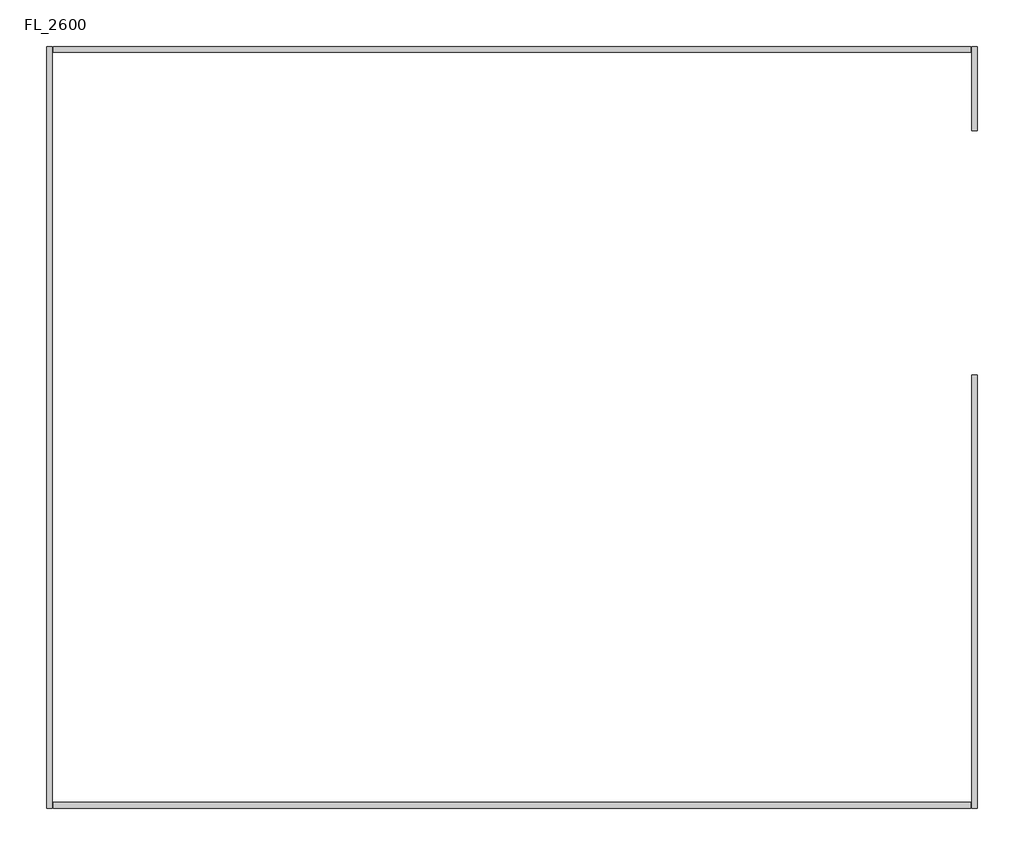
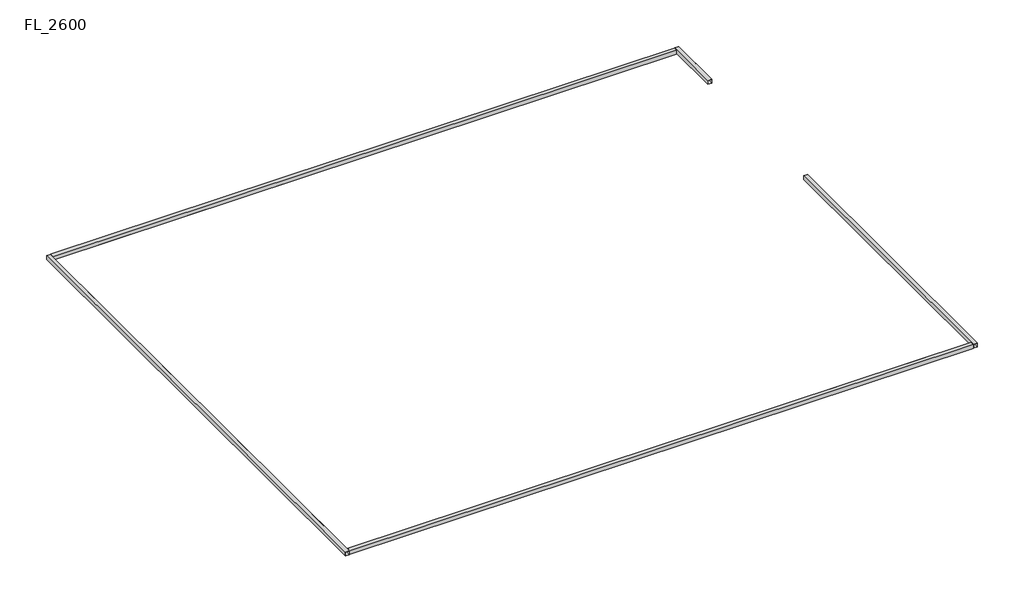
# One storey: 5 beams.
# Revit data of these elements (continued)
# Project information (continued)
#     \"af7cfdda-f71a-4a09-bb03-63e0c16d5d93-00152ffb\" ism_id=\"3a38a709-bfa8-404e-b889-5af5e78ea0bf\" /><element revit_id=\"af7cfdda-f71a-4a09-bb03-63e0c16d5d93-00152ffe\" ism_id=\"bebf0363-7e59-4a43-8f5b-502fcc4a338d\" /><element revit_id=\"af7cfdda-f71a-4a09-bb03-63e0c16d5d93-00153000\" ism_id=\"157fe154-0d28-4e8c-a143-e2896867fd28\" /><element revit_id=\"af7cfdda-f71a-4a09-bb03-63e0c16d5d93-00153002\" ism_id=\"1bf52bf8-7327-4d55-b5cd-bf7c9bf89688\" /><element revit_id=\"af7cfdda-f71a-4a09-bb03-63e0c16d5d93-00153005\" ism_id=\"7a0025bf-d54b-4614-9002-7bd4a82da90e\" /><element revit_id=\"af7cfdda-f71a-4a09-bb03-63e0c16d5d93-00153008\" ism_id=\"cad53638-8c8f-4a89-ab6f-d8a32131833b\" /><element revit_id=\"af7cfdda-f71a-4a09-bb03-63e0c16d5d93-0015300a\" ism_id=\"05672ccd-1a96-434c-8da1-7a706b3561f7\" /><element revit_id=\"af7cfdda-f71a-4a09-bb03-63e0c16d5d93-0015300c\" ism_id=\"bb809016-b2bb-4157-847e-1cca3692ba19\" /><element revit_id=\"af7cfdda-f71a-4a09-bb03-63e0c16d5d93-0015300f\" ism_id=\"720ed192-8aa7-46fd-9f7a-15d64351767c\" /><element revit_id=\"af7cfdda-f71a-4a09-bb03-63e0c16d5d93-00153011\" ism_id=\"9a47cdb9-976d-41f3-a5c3-5a7516a7763c\" /><element revit_id=\"af7cfdda-f71a-4a09-bb03-63e0c16d5d93-00153013\" ism_id=\"aba01787-c82b-453e-8db2-70277a34d5ad\" /><element revit_id=\"af7cfdda-f71a-4a09-bb03-63e0c16d5d93-00153015\" ism_id=\"f6b882e3-d64a-44b1-878c-9c00ee1fde86\" /><element revit_id=\"af7cfdda-f71a-4a09-bb03-63e0c16d5d93-00153017\" ism_id=\"95108815-490a-427a-aec1-8fcefc57c858\" /><element revit_id=\"af7cfdda-f71a-4a09-bb03-63e0c16d5d93-00153019\" ism_id=\"8fe55cf1-56b4-4a62-948a-d7f0c95bd04b\" /><element revit_id=\"af7cfdda-f71a-4a09-bb03-63e0c16d5d93-0015301b\" ism_id=\"b889bf8b-3bdd-410a-b11b-9ca69449d470\" /><element revit_id=\"af7cfdda-f71a-4a09-bb03-63e0c16d5d93-0015301d\" ism_id=\"ef8604de-de5b-45ec-9158-0b702e6ef713\" /><element revit_id=\"af7cfdda-f71a-4a09-bb03-63e0c16d5d93-0015301f\" ism_id=\"40ee286a-4bc9-4d4f-ba6d-fe1ac9da03cf\" /><element revit_id=\"af7cfdda-f71a-4a09-bb03-63e0c16d5d93-00153021\" ism_id=\"cc903f39-6bdf-4081-a56c-883169221735\" /><element revit_id=\"af7cfdda-f71a-4a09-bb03-63e0c16d5d93-00153023\" ism_id=\"0af04955-dcb6-4295-b3d4-7c432a233062\" /><element revit_id=\"af7cfdda-f71a-4a09-bb03-63e0c16d5d93-00153025\" ism_id=\"75a51549-6a04-4399-b818-f170a8c10286\" /><element revit_id=\"af7cfdda-f71a-4a09-bb03-63e0c16d5d93-00153027\" ism_id=\"7e183794-5c66-46bc-97f5-2df209b3286d\" /><element revit_id=\"af7cfdda-f71a-4a09-bb03-63e0c16d5d93-00153029\" ism_id=\"ed4a7448-29b0-44e3-8b6f-7310f83440ab\" /><element revit_id=\"af7cfdda-f71a-4a09-bb03-63e0c16d5d93-0015302b\" ism_id=\"fdb5eb17-b94e-40c1-b703-3ecb5e4efee4\" /><element revit_id=\"af7cfdda-f71a-4a09-bb03-63e0c16d5d93-0015302d\" ism_id=\"779397c1-65b7-447f-a72e-2a09308021ea\" /><element revit_id=\"af7cfdda-f71a-4a09-bb03-63e0c16d5d93-0015302f\" ism_id=\"7b409707-86c5-44e2-919e-92ad5bb9eb8b\" /><element revit_id=\"af7cfdda-f71a-4a09-bb03-63e0c16d5d93-00153031\" ism_id=\"d337c78b-590d-406c-bf20-6a3558821db1\" /><element revit_id=\"af7cfdda-f71a-4a09-bb03-63e0c16d5d93-00153033\" ism_id=\"c27f5f6d-8445-4415-853d-d316787bea6e\" /><element revit_id=\"af7cfdda-f71a-4a09-bb03-63e0c16d5d93-00153035\" ism_id=\"76036a55-3bab-417a-ba41-ec1335e2e2a7\" /><element revit_id=\"af7cfdda-f71a-4a09-bb03-63e0c16d5d93-00153037\" ism_id=\"24be638c-ff89-4616-8974-5b79c81e6e56\" /><element revit_id=\"af7cfdda-f71a-4a09-bb03-63e0c16d5d93-00153039\" ism_id=\"015f9f2c-2353-4795-b891-e4ee986f25f7\" /><element revit_id=\"af7cfdda-f71a-4a09-bb03-63e0c16d5d93-0015303b\" ism_id=\"91f8ddfb-c5b9-4f33-b141-a6edfbccf098\" /><element revit_id=\"af7cfdda-f71a-4a09-bb03-63e0c16d5d93-0015303d\" ism_id=\"78540364-1ba5-4f0c-95fb-ba8631e32695\" /><element revit_id=\"af7cfdda-f71a-4a09-bb03-63e0c16d5d93-0015303f\" ism_id=\"9d53e406-367b-4e3e-b5e8-d421731e1aab\" /><element revit_id=\"af7cfdda-f71a-4a09-bb03-63e0c16d5d93-00153041\" ism_id=\"24aa6051-1a20-4f08-8962-6f6f9ff4dc98\" /><element revit_id=\"af7cfdda-f71a-4a09-bb03-63e0c16d5d93-00153043\" ism_id=\"572a4144-5250-4962-a1b9-09502cda2774\" /><element revit_id=\"af7cfdda-f71a-4a09-bb03-63e0c16d5d93-00153045\" ism_id=\"1f486980-0be9-4aad-b32e-0608218bf68e\" /><element revit_id=\"af7cfdda-f71a-4a09-bb03-63e0c16d5d93-00153047\" ism_id=\"588ed856-d113-4521-b97c-a4d7ac7ba406\" /><element revit_id=\"af7cfdda-f71a-4a09-bb03-63e0c16d5d93-00153049\" ism_id=\"741942b7-995d-48cb-8401-4faec8ef8d15\" /><element revit_id=\"af7cfdda-f71a-4a09-bb03-63e0c16d5d93-0015304b\" ism_id=\"85254c30-08c9-46e3-acd6-6b5131f485ce\" /><element revit_id=\"af7cfdda-f71a-4a09-bb03-63e0c16d5d93-0015304e\" ism_id=\"2d57d6c0-67d8-48bd-b16f-8ef7edb485b1\" /><element revit_id=\"af7cfdda-f71a-4a09-bb03-63e0c16d5d93-00153050\" ism_id=\"57b4caff-473e-4ebc-b42c-d73ce4ca67d8\" /><element revit_id=\"af7cfdda-f71a-4a09-bb03-63e0c16d5d93-00153052\" ism_id=\"1adae240-a487-478c-a898-61bee40e7415\" /><element revit_id=\"af7cfdda-f71a-4a09-bb03-63e0c16d5d93-00153054\" ism_id=\"62613b5f-092e-4f63-86ac-d3e070a85bc5\" /><element revit_id=\"af7cfdda-f71a-4a09-bb03-63e0c16d5d93-00153056\" ism_id=\"6aecb1de-b991-4eed-80ad-e1b9ccc03a87\" /><element revit_id=\"af7cfdda-f71a-4a09-bb03-63e0c16d5d93-00153058\" ism_id=\"ecab5d8d-84d0-44a4-9549-bca959ac514b\" /><element revit_id=\"af7cfdda-f71a-4a09-bb03-63e0c16d5d93-0015305a\" ism_id=\"589f44ad-061b-46bc-91bd-bf9b1e708415\" /><element revit_id=\"af7cfdda-f71a-4a09-bb03-63e0c16d5d93-0015305c\" ism_id=\"bfa24af8-499f-45ff-9e9d-d5cc0761fed6\" /><element revit_id=\"af7cfdda-f71a-4a09-bb03-63e0c16d5d93-0015305e\" ism_id=\"8114f473-ca73-4cc8-b3e2-979f07368f66\" /><element revit_id=\"af7cfdda-f71a-4a09-bb03-63e0c16d5d93-00153060\" ism_id=\"4dde7439-2ac9-412f-a5f5-e9fd0f294ec8\" /><element revit_id=\"af7cfdda-f71a-4a09-bb03-63e0c16d5d93-00153062\" ism_id=\"661cc7d8-fd9c-4505-b43e-241bfd24b2d0\" /><element revit_id=\"af7cfdda-f71a-4a09-bb03-63e0c16d5d93-00153064\" ism_id=\"1e7f186f-1b55-4d4c-bf9f-18595049605e\" /><element revit_id=\"af7cfdda-f71a-4a09-bb03-63e0c16d5d93-00153066\" ism_id=\"ee968183-c9c6-4eab-86cf-0eda12de724b\" /><element revit_id=\"af7cfdda-f71a-4a09-bb03-63e0c16d5d93-00153068\" ism_id=\"5de1f319-cdd1-4b9a-8f8e-b86394effa22\" /><element revit_id=\"af7cfdda-f71a-4a09-bb03-63e0c16d5d93-0015306a\" ism_id=\"fa557a6c-2e39-4481-9eb5-5ede8fd31c49\" /><element revit_id=\"af7cfdda-f71a-4a09-bb03-63e0c16d5d93-0015306c\" ism_id=\"b2710e8e-0f5f-4e74-a366-aef04da22cd3\" /><element revit_id=\"af7cfdda-f71a-4a09-bb03-63e0c16d5d93-0015306e\" ism_id=\"5633c3b7-f903-46ee-b126-8a20a9a62c90\" /><element revit_id=\"af7cfdda-f71a-4a09-bb03-63e0c16d5d93-00153070\" ism_id=\"62796ef8-c4bb-4b9f-bd14-cc7392046eb4\" /><element revit_id=\"af7cfdda-f71a-4a09-bb03-63e0c16d5d93-00153072\" ism_id=\"db898ada-150e-4ff5-a9f8-16e27b46b754\" /><element revit_id=\"af7cfdda-f71a-4a09-bb03-63e0c16d5d93-00153075\" ism_id=\"d3965d2d-e119-4f6b-af8d-52c8a5397d36\" /><element revit_id=\"af7cfdda-f71a-4a09-bb03-63e0c16d5d93-00153077\" ism_id=\"063574e4-6319-4ba7-8e34-1638a1357d5f\" /><element revit_id=\"af7cfdda-f71a-4a09-bb03-63e0c16d5d93-00153079\" ism_id=\"6de69805-8980-44f0-9316-6d50d1b47cbb\" /><element revit_id=\"af7cfdda-f71a-4a09-bb03-63e0c16d5d93-0015307b\" ism_id=\"e5f77c5b-4806-4993-8875-6149db708e42\" /><element revit_id=\"af7cfdda-f71a-4a09-bb03-63e0c16d5d93-0015307d\" ism_id=\"a13071c9-c086-4896-95a6-a015bc531f25\" /><element revit_id=\"af7cfdda-f71a-4a09-bb03-63e0c16d5d93-0015307f\" ism_id=\"c9d216f9-adca-4752-b8c1-d779727505dd\" /><element revit_id=\"af7cfdda-f71a-4a09-bb03-63e0c16d5d93-00153081\" ism_id=\"5b167621-3850-4169-8bee-1e0420bf6050\" /><element revit_id=\"af7cfdda-f71a-4a09-bb03-63e0c16d5d93-00153083\" ism_id=\"09cf76ae-a083-4203-a622-7e9424374f66\" /><element revit_id=\"af7cfdda-f71a-4a09-bb03-63e0c16d5d93-00153085\" ism_id=\"14063b50-058d-464a-aa08-369865983eeb\" /><element revit_id=\"af7cfdda-f71a-4a09-bb03-63e0c16d5d93-00153087\" ism_id=\"add5837f-63be-4349-b708-9f4051059e25\" /><element revit_id=\"af7cfdda-f71a-4a09-bb03-63e0c16d5d93-00153089\" ism_id=\"b4c60bd3-61cb-423f-916a-fa2b71585228\" /><element revit_id=\"af7cfdda-f71a-4a09-bb03-63e0c16d5d93-0015308b\" ism_id=\"6251d90e-381f-4771-818c-f7465ae91864\" /><element revit_id=\"af7cfdda-f71a-4a09-bb03-63e0c16d5d93-0015308d\" ism_id=\"7693be9d-48ca-4005-bed4-90e9c08d3a38\" /><element revit_id=\"af7cfdda-f71a-4a09-bb03-63e0c16d5d93-0015308f\" ism_id=\"a6a39ca9-cd56-43ba-bfe8-2cf3b78878cc\" /><element revit_id=\"af7cfdda-f71a-4a09-bb03-63e0c16d5d93-00153091\" ism_id=\"1a3956c4-77bb-4ccc-a12d-c3514cf365d4\" /><element revit_id=\"af7cfdda-f71a-4a09-bb03-63e0c16d5d93-00153093\" ism_id=\"2ffa7a89-8ee9-470a-b3d8-7c27f566e226\" /><element revit_id=\"af7cfdda-f71a-4a09-bb03-63e0c16d5d93-00153095\" ism_id=\"e865b460-944f-4057-a6e8-4e39cb88d97d\" /><element revit_id=\"af7cfdda-f71a-4a09-bb03-63e0c16d5d93-00153097\" ism_id=\"69410bb9-8440-4a88-9151-b5459095fe2e\" /><element revit_id=\"af7cfdda-f71a-4a09-bb03-63e0c16d5d93-00153099\" ism_id=\"1efae87b-0246-432c-a428-82c87fb3929c\" /><element revit_id=\"af7cfdda-f71a-4a09-bb03-63e0c16d5d93-0015309b\" ism_id=\"e1d5fb57-3b5d-4a32-bccb-cea278671f2f\" /><element revit_id=\"af7cfdda-f71a-4a09-bb03-63e0c16d5d93-0015309d\" ism_id=\"c74a7061-f4b2-41b5-b3ff-caf6cf9dfffd\" /><element revit_id=\"af7cfdda-f71a-4a09-bb03-63e0c16d5d93-0015309f\" ism_id=\"aa777ec3-1257-49eb-b597-fbab7bda8b11\" /><element revit_id=\"af7cfdda-f71a-4a09-bb03-63e0c16d5d93-001530a1\" ism_id=\"7420a67b-bb48-477d-823a-c473ce92c083\" /><element revit_id=\"af7cfdda-f71a-4a09-bb03-63e0c16d5d93-001530a3\" ism_id=\"1ee9340a-8778-4cd6-be2d-57fb5fe16e45\" /><element revit_id=\"af7cfdda-f71a-4a09-bb03-63e0c16d5d93-001530a5\" ism_id=\"3216ac21-29b0-45a7-a070-99a114df4980\" /><element revit_id=\"af7cfdda-f71a-4a09-bb03-63e0c16d5d93-001530a7\" ism_id=\"dce9c5c3-a57a-4091-8398-cace2e63f290\" /><element revit_id=\"af7cfdda-f71a-4a09-bb03-63e0c16d5d93-001530a9\" ism_id=\"dcadcd2e-1b12-41e7-a9d5-5d99303c7e51\" /><element revit_id=\"af7cfdda-f71a-4a09-bb03-63e0c16d5d93-001530ab\" ism_id=\"ed4bf433-a5ea-40d4-8551-b735160eed03\" /><element revit_id=\"af7cfdda-f71a-4a09-bb03-63e0c16d5d93-001530ad\" ism_id=\"2cd91197-39b9-4301-8775-b1530f8812f8\" /><element revit_id=\"af7cfdda-f71a-4a09-bb03-63e0c16d5d93-001530af\" ism_id=\"53460b48-5382-4fff-98f2-ab500700bbca\" /><element revit_id=\"af7cfdda-f71a-4a09-bb03-63e0c16d5d93-001530b1\" ism_id=\"0d733cb9-b11e-45a1-89e1-53989b2ba4d5\" /><element revit_id=\"af7cfdda-f71a-4a09-bb03-63e0c16d5d93-001530b3\" ism_id=\"9b6990cb-bf48-452d-9572-952a8acd923b\" /><element revit_id=\"af7cfdda-f71a-4a09-bb03-63e0c16d5d93-001530b5\" ism_id=\"edb53df5-f0f8-45af-a38d-8c910b94c4aa\" /><element revit_id=\"af7cfdda-f71a-4a09-bb03-63e0c16d5d93-001530b7\" ism_id=\"a42a99cd-d791-460b-b7db-769eef45d4ee\" /><element revit_id=\"af7cfdda-f71a-4a09-bb03-63e0c16d5d93-001530b9\" ism_id=\"473eafff-0971-4b1a-8b61-a7662a5d0782\" /><element revit_id=\"af7cfdda-f71a-4a09-bb03-63e0c16d5d93-001530bb\" ism_id=\"b801d819-54a6-4fd3-91e7-5d49978bee50\" /><element revit_id=\"af7cfdda-f71a-4a09-bb03-63e0c16d5d93-001530bd\" ism_id=\"aa72d39c-13a9-4733-9528-98e90ae2a493\" /><element revit_id=\"af7cfdda-f71a-4a09-bb03-63e0c16d5d93-001530c0\" ism_id=\"e50950ab-c982-40e9-a130-a8fe9c5071aa\" /><element revit_id=\"af7cfdda-f71a-4a09-bb03-63e0c16d5d93-001530c3\" ism_id=\"caa8c896-9dda-4bb9-b942-fab7d7988525\" /><element revit_id=\"af7cfdda-f71a-4a09-bb03-63e0c16d5d93-001530c5\" ism_id=\"45f4fe9a-436c-4b4d-a48d-573edf59a390\" /><element revit_id=\"af7cfdda-f71a-4a09-bb03-63e0c16d5d93-001530c7\" ism_id=\"eb513efb-1058-4d3f-8f19-56219176a71a\" /><element revit_id=\"af7cfdda-f71a-4a09-bb03-63e0c16d5d93-001530c9\" ism_id=\"537abf12-3423-4f70-8613-a81d434152a6\" /><element revit_id=\"af7cfdda-f71a-4a09-bb03-63e0c16d5d93-001530cb\" ism_id=\"683f9f6d-960e-4ae9-ad7f-39eee39c3d47\" /><element revit_id=\"af7cfdda-f71a-4a09-bb03-63e0c16d5d93-001530cd\" ism_id=\"2ceed54c-aecf-4b75-a53e
#     -cfd758078946\" /><element revit_id=\"af7cfdda-f71a-4a09-bb03-63e0c16d5d93-001530cf\" ism_id=\"46a5ded9-4fed-43a0-a06e-bb0fce603002\" /><element revit_id=\"af7cfdda-f71a-4a09-bb03-63e0c16d5d93-001530d1\" ism_id=\"62d05a0c-55f2-4c29-a355-b77f91c84c50\" /><element revit_id=\"af7cfdda-f71a-4a09-bb03-63e0c16d5d93-001530d3\" ism_id=\"eac0c420-7041-45a3-ad98-0cab4f5d8155\" /><element revit_id=\"af7cfdda-f71a-4a09-bb03-63e0c16d5d93-001530d5\" ism_id=\"9f5beb51-429a-4c7b-aa2e-ad2efe601ed6\" /><element revit_id=\"af7cfdda-f71a-4a09-bb03-63e0c16d5d93-001530d7\" ism_id=\"4613af3e-a189-4781-a937-106d789655c9\" /><element revit_id=\"af7cfdda-f71a-4a09-bb03-63e0c16d5d93-001530d9\" ism_id=\"71402e21-51c1-43b7-b8cc-75d2aba247eb\" /><element revit_id=\"af7cfdda-f71a-4a09-bb03-63e0c16d5d93-001530db\" ism_id=\"89101b83-9b84-4f11-b026-90cd564a3900\" /><element revit_id=\"af7cfdda-f71a-4a09-bb03-63e0c16d5d93-001530dd\" ism_id=\"37670781-ce23-4ce1-992b-7a400613c37b\" /><element revit_id=\"af7cfdda-f71a-4a09-bb03-63e0c16d5d93-001530df\" ism_id=\"2316856d-18eb-466b-8ab8-114816378db0\" /><element revit_id=\"af7cfdda-f71a-4a09-bb03-63e0c16d5d93-001530e2\" ism_id=\"da4f1597-5b5a-43a6-aa94-e478ffd6cfc7\" /><element revit_id=\"af7cfdda-f71a-4a09-bb03-63e0c16d5d93-001530e5\" ism_id=\"60805764-efb2-4434-8d81-aed3c3ed3c1b\" /><element revit_id=\"af7cfdda-f71a-4a09-bb03-63e0c16d5d93-001530e8\" ism_id=\"34e34ebb-6481-4bfb-b3d0-cb52295ff652\" /><element revit_id=\"af7cfdda-f71a-4a09-bb03-63e0c16d5d93-001530eb\" ism_id=\"dd5c4d73-1406-4c40-a955-5f9c52d01161\" /><element revit_id=\"af7cfdda-f71a-4a09-bb03-63e0c16d5d93-001530ed\" ism_id=\"cf8abc6b-638f-4bd5-8b66-615be032e220\" /><element revit_id=\"af7cfdda-f71a-4a09-bb03-63e0c16d5d93-001530f0\" ism_id=\"56ce8857-0c24-48d5-82f2-459e263998e2\" /><element revit_id=\"af7cfdda-f71a-4a09-bb03-63e0c16d5d93-001530f2\" ism_id=\"a1f000e8-ea08-442b-8a96-da7657653fd5\" /><element revit_id=\"af7cfdda-f71a-4a09-bb03-63e0c16d5d93-001530f4\" ism_id=\"2625e954-f7fb-41eb-b9bd-1b615ef945fc\" /><element revit_id=\"af7cfdda-f71a-4a09-bb03-63e0c16d5d93-001530f6\" ism_id=\"48469362-393c-4deb-bbb2-ad00180a23fb\" /><element revit_id=\"af7cfdda-f71a-4a09-bb03-63e0c16d5d93-001530f8\" ism_id=\"8e650f6f-0906-45a9-8fb8-35680155d6db\" /><element revit_id=\"af7cfdda-f71a-4a09-bb03-63e0c16d5d93-001530fb\" ism_id=\"f84acaf6-20a1-4df6-afed-1dc07fd0b2e9\" /><element revit_id=\"af7cfdda-f71a-4a09-bb03-63e0c16d5d93-001530fe\" ism_id=\"72816c7e-9128-47f4-b46a-ee567a2a03d6\" /><element revit_id=\"af7cfdda-f71a-4a09-bb03-63e0c16d5d93-00153100\" ism_id=\"c95ab0f8-b4bf-4b7c-bd1d-0423c8ac725a\" /><element revit_id=\"af7cfdda-f71a-4a09-bb03-63e0c16d5d93-00153102\" ism_id=\"32fd4119-6673-4973-aef2-b39ef90310e5\" /><element revit_id=\"af7cfdda-f71a-4a09-bb03-63e0c16d5d93-00153104\" ism_id=\"fd2aa4a6-d123-4100-85b9-db27c20cf6bc\" /><element revit_id=\"af7cfdda-f71a-4a09-bb03-63e0c16d5d93-00153106\" ism_id=\"e00fdefa-e77c-4406-9dbe-3c9122259821\" /><element revit_id=\"af7cfdda-f71a-4a09-bb03-63e0c16d5d93-00153108\" ism_id=\"25e5b79e-07c2-4ffa-a7a9-bf039dd2ad78\" /><element revit_id=\"af7cfdda-f71a-4a09-bb03-63e0c16d5d93-0015310b\" ism_id=\"720021d4-ca74-47c0-9c64-7d0854fa39f5\" /><element revit_id=\"af7cfdda-f71a-4a09-bb03-63e0c16d5d93-0015310d\" ism_id=\"ea922120-0cff-4f8d-a5c2-2841c031873e\" /><element revit_id=\"af7cfdda-f71a-4a09-bb03-63e0c16d5d93-0015310f\" ism_id=\"9d07ca73-3a65-44fe-ab61-476d8d1352d1\" /><element revit_id=\"af7cfdda-f71a-4a09-bb03-63e0c16d5d93-00153111\" ism_id=\"68a2fb30-d213-40c7-a166-dad5a20bd269\" /><element revit_id=\"af7cfdda-f71a-4a09-bb03-63e0c16d5d93-00153113\" ism_id=\"06119775-28f9-44f0-a265-5c57029016d1\" /><element revit_id=\"af7cfdda-f71a-4a09-bb03-63e0c16d5d93-00153115\" ism_id=\"ca133383-8253-4d07-aa92-f507fbb2ee47\" /><element revit_id=\"af7cfdda-f71a-4a09-bb03-63e0c16d5d93-00153117\" ism_id=\"6f4a7c07-4bd3-4c99-b1e4-110c964ccc07\" /><element revit_id=\"af7cfdda-f71a-4a09-bb03-63e0c16d5d93-00153119\" ism_id=\"ee1f865b-98a9-4ff1-a84c-52926e8f3566\" /><element revit_id=\"af7cfdda-f71a-4a09-bb03-63e0c16d5d93-0015311b\" ism_id=\"4fd7bd5c-7c46-4e79-a72b-dab4a1d98f33\" /><element revit_id=\"af7cfdda-f71a-4a09-bb03-63e0c16d5d93-0015311e\" ism_id=\"9ca0cac6-aaff-412a-b9c1-a8be985bc44a\" /><element revit_id=\"af7cfdda-f71a-4a09-bb03-63e0c16d5d93-00153121\" ism_id=\"73123639-76b5-46f0-a49e-b26af36d93b1\" /><element revit_id=\"af7cfdda-f71a-4a09-bb03-63e0c16d5d93-00153123\" ism_id=\"f74e8cb9-a93d-4aaa-985b-c0ed9befad19\" /><element revit_id=\"af7cfdda-f71a-4a09-bb03-63e0c16d5d93-00153126\" ism_id=\"5778daa1-b4cb-4cc3-9b7d-323562a47fba\" /><element revit_id=\"af7cfdda-f71a-4a09-bb03-63e0c16d5d93-00153129\" ism_id=\"2d7457d2-8978-4c95-9056-ebbaed3263eb\" /><element revit_id=\"af7cfdda-f71a-4a09-bb03-63e0c16d5d93-0015312c\" ism_id=\"48b420ce-6767-430a-aadc-695c25361a2d\" /><element revit_id=\"af7cfdda-f71a-4a09-bb03-63e0c16d5d93-0015312e\" ism_id=\"fc34038c-136d-4d55-b951-9cc35899fd33\" /><element revit_id=\"af7cfdda-f71a-4a09-bb03-63e0c16d5d93-00153130\" ism_id=\"e7a25938-3b91-4519-a48d-86fdd79489d5\" /><element revit_id=\"af7cfdda-f71a-4a09-bb03-63e0c16d5d93-00153133\" ism_id=\"c81dfd8c-579c-4d77-ab89-bf1f415d9cc6\" /><element revit_id=\"af7cfdda-f71a-4a09-bb03-63e0c16d5d93-00153136\" ism_id=\"5756a4b4-84ca-418c-b9f6-2d2370afca2f\" /><element revit_id=\"af7cfdda-f71a-4a09-bb03-63e0c16d5d93-0015313a\" ism_id=\"09a9cede-a757-4d8e-a722-6140af98bc61\" /><element revit_id=\"af7cfdda-f71a-4a09-bb03-63e0c16d5d93-0015313d\" ism_id=\"ac9b583c-7f63-4351-8b69-3967279b234c\" /><element revit_id=\"af7cfdda-f71a-4a09-bb03-63e0c16d5d93-00153140\" ism_id=\"1a52584d-6b21-4de6-bb42-5b9bdd6f24e9\" /><element revit_id=\"af7cfdda-f71a-4a09-bb03-63e0c16d5d93-00153143\" ism_id=\"6c2e2bc0-8432-4c98-9292-cbb2182bd4b0\" /><element revit_id=\"af7cfdda-f71a-4a09-bb03-63e0c16d5d93-00153145\" ism_id=\"644bb900-7654-42c5-a9b7-996a2197f6d0\" /><element revit_id=\"af7cfdda-f71a-4a09-bb03-63e0c16d5d93-00153148\" ism_id=\"a1bca0bd-75db-464c-b27a-2a69d9b4ad3d\" /><element revit_id=\"af7cfdda-f71a-4a09-bb03-63e0c16d5d93-0015314a\" ism_id=\"ea29955b-34f2-409a-aefa-e6adfe75349e\" /><element revit_id=\"af7cfdda-f71a-4a09-bb03-63e0c16d5d93-0015314d\" ism_id=\"800fef33-e5e1-422c-b708-e9394bbeefcc\" /><element revit_id=\"af7cfdda-f71a-4a09-bb03-63e0c16d5d93-0015314f\" ism_id=\"86259dca-8773-4253-ac56-e71252267c8a\" /><element revit_id=\"af7cfdda-f71a-4a09-bb03-63e0c16d5d93-00153152\" ism_id=\"d15a0ad2-db9f-420d-bea3-41a78a0eb330\" /><element revit_id=\"af7cfdda-f71a-4a09-bb03-63e0c16d5d93-00153155\" ism_id=\"bd27f420-df49-4abe-bd96-8e48e7f4efcb\" /><element revit_id=\"af7cfdda-f71a-4a09-bb03-63e0c16d5d93-00153157\" ism_id=\"5d451f94-860d-4cc3-a4fa-51a9f3126e33\" /><element revit_id=\"af7cfdda-f71a-4a09-bb03-63e0c16d5d93-0015315a\" ism_id=\"4234158a-994a-492b-85da-6108709b7232\" /><element revit_id=\"af7cfdda-f71a-4a09-bb03-63e0c16d5d93-0015315c\" ism_id=\"ca24c92d-986b-417f-812f-024ab15e24c8\" /><element revit_id=\"af7cfdda-f71a-4a09-bb03-63e0c16d5d93-0015315f\" ism_id=\"699ec3b0-0151-4110-b054-14418651f324\" /><element revit_id=\"af7cfdda-f71a-4a09-bb03-63e0c16d5d93-00153161\" ism_id=\"38ecdeac-3d85-48dd-82c1-53fe93f49beb\" /><element revit_id=\"af7cfdda-f71a-4a09-bb03-63e0c16d5d93-00153163\" ism_id=\"1340aefd-b79c-4264-8a49-d0a0504eff8c\" /><element revit_id=\"af7cfdda-f71a-4a09-bb03-63e0c16d5d93-00153165\" ism_id=\"1b6167c2-fb26-4b8d-916b-d835d89896e7\" /><element revit_id=\"af7cfdda-f71a-4a09-bb03-63e0c16d5d93-00153167\" ism_id=\"290d3d83-57eb-4125-aecb-a977a5fcf5ca\" /><element revit_id=\"af7cfdda-f71a-4a09-bb03-63e0c16d5d93-00153169\" ism_id=\"105c9b97-1c70-4237-82ac-8404a3e8e6a6\" /><element revit_id=\"af7cfdda-f71a-4a09-bb03-63e0c16d5d93-0015316c\" ism_id=\"1726c5bb-05e2-4959-9da2-4227f0219f00\" /><element revit_id=\"af7cfdda-f71a-4a09-bb03-63e0c16d5d93-0015316e\" ism_id=\"d919ee9c-caed-4119-b451-e3644db952c8\" /><element revit_id=\"af7cfdda-f71a-4a09-bb03-63e0c16d5d93-00153170\" ism_id=\"1b1fab26-60c4-40ed-b31b-b177eda246ce\" /><element revit_id=\"af7cfdda-f71a-4a09-bb03-63e0c16d5d93-00153172\" ism_id=\"ea9b5221-a1f2-4796-8cca-f7872ab69cbd\" /><element revit_id=\"af7cfdda-f71a-4a09-bb03-63e0c16d5d93-00153174\" ism_id=\"660b40b2-06fb-4b62-b987-28a171e473fe\" /><element revit_id=\"af7cfdda-f71a-4a09-bb03-63e0c16d5d93-00153176\" ism_id=\"767be0d9-c5ba-4ad3-a52d-efd60031fc9a\" /><element revit_id=\"af7cfdda-f71a-4a09-bb03-63e0c16d5d93-00153178\" ism_id=\"6fbe93ce-4ed7-4596-88fc-71dafe48803e\" /><element revit_id=\"af7cfdda-f71a-4a09-bb03-63e0c16d5d93-0015317a\" ism_id=\"27d7b093-4eb7-47aa-b123-5388a6327d7f\" /><element revit_id=\"af7cfdda-f71a-4a09-bb03-63e0c16d5d93-0015317c\" ism_id=\"9073a947-5952-42fe-b37a-cdfed3ca30c7\" /><element revit_id=\"af7cfdda-f71a-4a09-bb03-63e0c16d5d93-0015317e\" ism_id=\"1888f060-aa3c-4494-8f30-a80ca2311216\" /><element revit_id=\"af7cfdda-f71a-4a09-bb03-63e0c16d5d93-00153181\" ism_id=\"c0491dc2-5df2-4c14-b988-e117f6f511a2\" /><element revit_id=\"af7cfdda-f71a-4a09-bb03-63e0c16d5d93-00153184\" ism_id=\"4f44b9aa-c092-46fe-bf9b-2d1be872d419\" /><element revit_id=\"af7cfdda-f71a-4a09-bb03-63e0c16d5d93-00153186\" ism_id=\"eb560801-76cf-40a8-a181-31cd32aca14f\" /><element revit_id=\"af7cfdda-f71a-4a09-bb03-63e0c16d5d93-00153189\" ism_id=\"8d1e5f00-41d5-42c1-9b4f-a8c2eb689a72\" /><element revit_id=\"af7cfdda-f71a-4a09-bb03-63e0c16d5d93-0015318b\" ism_id=\"caf6c2dc-0e9e-46a9-a3e1-71316081ff61\" /><element revit_id=\"af7cfdda-f71a-4a09-bb03-63e0c16d5d93-0015318d\" ism_id=\"4d149f88-f5b9-4943-8765-090324e0a65d\" /><element revit_id=\"af7cfdda-f71a-4a09-bb03-63e0c16d5d93-0015318f\" ism_id=\"75865cf2-3adc-4a52-a778-fc6fb65fcdcb\" /><element revit_id=\"af7cfdda-f71a-4a09-bb03-63e0c16d5d93-00153191\" ism_id=\"f9320017-2083-48f1-8aff-e6ba958fb1c5\" /><element revit_id=\"af7cfdda-f71a-4a09-bb03-63e0c16d5d93-00153193\" ism_id=\"38a61c12-98f2-47b1-843d-8351040e24d2\" /><element revit_id=\"af7cfdda-f71a-4a09-bb03-63e0c16d5d93-00153196\" ism_id=\"af709a9c-b664-480b-be0d-fb01aac630f2\" /><element revit_id=\"af7cfdda-f71a-4a09-bb03-63e0c16d5d93-00153199\" ism_id=\"a4c2867c-ca2a-4112-b86c-4e6563e3dc63\" /><element revit_id=\"14a48413-84c4-4e00-9e64-4f618415469a-0013ce74\" ism_id=\"F2ADF140-E21A-4820-8170-6F63D956DCAD\" /><element revit_id=\"14a48413-84c4-4e00-9e64-4f618415469a-0013ce74\" ism_id=\"B35A310E-4F33-462b-819C-3ADD300C0CEB\" /><element revit_id=\"14a48413-84c4-4e00-9e64-4f618415469a-0013ce74\" ism_id=\"711054EC-0DB2-46e3-AD20-004560300C00\" /><element revit_id=\"14a48413-84c4-4e00-9e64-4f618415469a-0013ce6e\" ism_id=\"B5C54EC9-8EBD-4860-AB72-EF5791AED394\" /><element revit_id=\"14a48413-84c4-4e00-9e64-4f618415469a-0013e793\" ism_id=\"0A7B8D02-9EA4-4aa9-A41A-E30BB5B6B6C5\" /><element revit_id=\"14a48413-84c4-4e00-9e64-4f618415469a-0013e793\" ism_id=\"714BBD27-DB58-47da-B54C-5806291C2D3C\" /><element revit_id=\"14a48413-84c4-4e00-9e64-4f618415469a-0013e793\" ism_id=\"F36E62C1-13EE-4807-A3C1-899E23E0BEDE\" /><element revit_id=\"14a48413-84c4-4e00-9e64-4f618415469a-0013e793\" ism_id=\"F5448801-679E-44d6-8F46-E676344F8165\" /><element revit_id=\"14a48413-84c4-4e00-9e64-4f618415469a-0013e793\" ism_id=\"846DCB0C-E06B-4978-9D43-E1CC0FDE7595\" /><element revit_id=\"14a48413-84c4-4e00-9e64-4f618415469a-0013e793\" ism_id=\"2ADF82B8-986D-4f44-85DE-89D921292160\" /><element revit_id=\"14a48413-84c4-4e00-9e64-4f618415469a-0013e793\" ism_id=\"7AF371ED-051B-4a30-8826-11F11C212B73\" /><element revit_id=\"14a48413-84c4-4e00-9e64-4f618415469a-0013e793\" ism_id=\"2FE74006-ADDA-412f-A522-853919E62B4D\" /><element revit_id=\"14a48413-84c4-4e00-9e64-4f618415469a-0013e793\" ism_id=\"09B63641-D581-4a6c-A18E-54C17EC989A4\" /><element revit_id=\"14a48413-84c4-4e00-9e64-4f618415469a-0013e793\" ism_id=\"0DD6B52A-77D0-45a1-82B1-8236ED57078C\" /><element revit_id=\"14a48413-84c4-4e00-9e64-4f618415469a-0013e793\" ism_id=\"35D311D2-DEB8-4469-97DE-110B6DF5B84D\" /><element revit_id=\"14a48413-84c4-4e00-9e64-4f618415469a-0013e79
#     3\" ism_id=\"0D3CCDE5-CFF9-431b-A4BD-01BF6636D6BD\" /><element revit_id=\"14a48413-84c4-4e00-9e64-4f618415469a-0013e793\" ism_id=\"C62B2A5B-024A-47ac-B030-C17A67E64A7B\" /><element revit_id=\"14a48413-84c4-4e00-9e64-4f618415469a-0013e793\" ism_id=\"944C6E43-E607-48c3-8358-9E6CB88346E7\" /><element revit_id=\"14a48413-84c4-4e00-9e64-4f618415469a-0013e793\" ism_id=\"A4B1F42D-B1C2-4ad2-8AD6-DB0D5E05998D\" /><element revit_id=\"14a48413-84c4-4e00-9e64-4f618415469a-0013e793\" ism_id=\"007E6C70-1139-4b48-B003-C76FAD4C249A\" /><element revit_id=\"14a48413-84c4-4e00-9e64-4f618415469a-0013e793\" ism_id=\"9941AC94-F03A-464c-9912-04590E0C31E0\" /><element revit_id=\"14a48413-84c4-4e00-9e64-4f618415469a-0013e793\" ism_id=\"CFD98B8D-8FF4-4e71-A909-0FE7DBCE924E\" /><element revit_id=\"14a48413-84c4-4e00-9e64-4f618415469a-0013e793\" ism_id=\"58262161-98E6-45c8-B2BD-4508105FF662\" /><element revit_id=\"14a48413-84c4-4e00-9e64-4f618415469a-0013e793\" ism_id=\"66AB4841-610A-4883-97F7-1282A56484E1\" /><element revit_id=\"14a48413-84c4-4e00-9e64-4f618415469a-0013e793\" ism_id=\"D2B324BE-BBD6-49da-9730-60EA7AD4D3A0\" /><element revit_id=\"14a48413-84c4-4e00-9e64-4f618415469a-0013e793\" ism_id=\"92A8ECE7-C053-46b1-92ED-F2C041617E7B\" /><element revit_id=\"14a48413-84c4-4e00-9e64-4f618415469a-0013e793\" ism_id=\"B4C4BDB0-65C4-4016-9C78-DBD77E229523\" /><element revit_id=\"14a48413-84c4-4e00-9e64-4f618415469a-0013e793\" ism_id=\"57270646-162F-4c83-BDB7-A5FBEA9120BD\" /><element revit_id=\"14a48413-84c4-4e00-9e64-4f618415469a-0013e793\" ism_id=\"BDEF733F-00AA-4eee-B6C6-50229FC1D236\" /><element revit_id=\"14a48413-84c4-4e00-9e64-4f618415469a-0013e793\" ism_id=\"84A94E1E-3074-40f4-9690-97191755F019\" /><element revit_id=\"14a48413-84c4-4e00-9e64-4f618415469a-0013e793\" ism_id=\"8A7D913D-7967-4718-912D-B83DF0AD2EDD\" /><element revit_id=\"14a48413-84c4-4e00-9e64-4f618415469a-0013e793\" ism_id=\"83553D70-90FA-469c-B5C3-EF03F3FC6475\" /><element revit_id=\"14a48413-84c4-4e00-9e64-4f618415469a-0013e793\" ism_id=\"6880C1E4-C50B-4c1b-B61C-23F2D8C46873\" /><element revit_id=\"14a48413-84c4-4e00-9e64-4f618415469a-0013e793\" ism_id=\"08594C43-CD40-47de-A3BA-8BFB47F64994\" /><element revit_id=\"14a48413-84c4-4e00-9e64-4f618415469a-0013e793\" ism_id=\"7D2E11FA-A5E1-4434-B9BE-AABA1A16CA03\" /><element revit_id=\"14a48413-84c4-4e00-9e64-4f618415469a-0013e793\" ism_id=\"D892DFA4-5441-4ad2-A390-253492293B1B\" /><element revit_id=\"14a48413-84c4-4e00-9e64-4f618415469a-0013e793\" ism_id=\"E5A32FE6-89C4-49f1-B3B9-1CABE7C48A4D\" /><element revit_id=\"14a48413-84c4-4e00-9e64-4f618415469a-0013e793\" ism_id=\"8AE872C2-5DBE-47c5-934B-7E964A84B589\" /><element revit_id=\"14a48413-84c4-4e00-9e64-4f618415469a-0013e793\" ism_id=\"3C847B60-488A-4604-A400-16A3A65E919B\" /><element revit_id=\"14a48413-84c4-4e00-9e64-4f618415469a-0013e793\" ism_id=\"DBEC432A-3F7B-4266-AD99-2A937DC70BCF\" /><element revit_id=\"14a48413-84c4-4e00-9e64-4f618415469a-0013e793\" ism_id=\"59403DD6-7A51-48aa-A3BE-962457E6F10E\" /><element revit_id=\"14a48413-84c4-4e00-9e64-4f618415469a-0013e793\" ism_id=\"11CDDF5D-38B6-43b2-A291-FC188BE232BC\" /><element revit_id=\"14a48413-84c4-4e00-9e64-4f618415469a-0013e793\" ism_id=\"10BF2843-EFC9-4136-933C-5B270D970277\" /><element revit_id=\"14a48413-84c4-4e00-9e64-4f618415469a-0013e793\" ism_id=\"E1B09A9C-F6C6-47d9-976B-E313C0E3F52B\" /><element revit_id=\"14a48413-84c4-4e00-9e64-4f618415469a-0013e793\" ism_id=\"A3A22EC3-26C8-4588-A0AB-AFAE02DF267E\" /><element revit_id=\"14a48413-84c4-4e00-9e64-4f618415469a-0013e793\" ism_id=\"114828FC-BDC1-4343-9119-BCB5395DAA64\" /><element revit_id=\"14a48413-84c4-4e00-9e64-4f618415469a-0013e793\" ism_id=\"797626F9-3558-4623-826F-15FB93088CB3\" /><element revit_id=\"14a48413-84c4-4e00-9e64-4f618415469a-0013e793\" ism_id=\"4BF369CD-DF09-4346-96CB-C6C6380A2599\" /><element revit_id=\"14a48413-84c4-4e00-9e64-4f618415469a-0013e793\" ism_id=\"722B46BA-61C4-44a1-9ECF-325B60B6688D\" /><element revit_id=\"14a48413-84c4-4e00-9e64-4f618415469a-0013e793\" ism_id=\"C33DBE84-19C1-4379-AB6E-A41F7420F18C\" /><element revit_id=\"14a48413-84c4-4e00-9e64-4f618415469a-0013e793\" ism_id=\"1F2D3B75-66F2-4d88-A1DD-647969477B86\" /><element revit_id=\"14a48413-84c4-4e00-9e64-4f618415469a-0013e793\" ism_id=\"DFBF96B2-410A-4f39-80C4-D8CF78561C93\" /><element revit_id=\"14a48413-84c4-4e00-9e64-4f618415469a-0013e793\" ism_id=\"D6793CD3-AB64-417c-9C28-8B18A0A2D336\" /><element revit_id=\"14a48413-84c4-4e00-9e64-4f618415469a-0013e793\" ism_id=\"90884AC0-EA00-4caa-86E1-E6B886FD90ED\" /><element revit_id=\"14a48413-84c4-4e00-9e64-4f618415469a-0013e793\" ism_id=\"64BC7B89-F7C8-4dae-A5C8-F10DF9E5F6BA\" /><element revit_id=\"14a48413-84c4-4e00-9e64-4f618415469a-0013e793\" ism_id=\"D82E4D85-2728-40e5-9F60-1C7FB2990D78\" /><element revit_id=\"14a48413-84c4-4e00-9e64-4f618415469a-0013e793\" ism_id=\"1E6D05B9-BF84-4669-AA27-948ADA1D511E\" /><element revit_id=\"14a48413-84c4-4e00-9e64-4f618415469a-0013e793\" ism_id=\"73608CB2-EB94-466e-883D-814030EF49D6\" /><element revit_id=\"14a48413-84c4-4e00-9e64-4f618415469a-0013e793\" ism_id=\"4EAF07EF-4E08-4065-9F08-BF69D4413867\" /><element revit_id=\"14a48413-84c4-4e00-9e64-4f618415469a-0013e0e9\" ism_id=\"05D74241-6318-4cac-95F5-7B878260D5B5\" /></element_binding><reinforcement_properties /><operation_settings><coordinate_mapping x=\"0\" y=\"0\" z=\"0\" /></operation_settings></ism>"
#   Building Name = "FIRE WATER PUMP BUILDING"
#   Project Status = "Project Status"
#   Client Name = "현대엔지니어링"
#   Project Address = "서울시 종로구 율곡로 75(계동)"
#   Project Name = "TAKHIATASH POWER PLANT EFFICIENCY IMPROVEMENT PROJECT / 우즈베키스탄"
#   Project Number = "BEUZ1602"
#   F01) Building Name = "FIRE WATER PUMP BUILDING"
#   F11) Project Building Tag_Type-1 = "BI aWBS"
#   F12) Project Building Tag_Type-2 = "BI aWBS"
#   F13) Project Facility Code = "621"
#   F21) Structural Type = "STEEL"
#   F31) Standard Building Code = "E204"
#   F41) Discipline = "Architecture"
#   F51) Plan Start Date-Engineering = "2018-01-01"
#   F52) Plan Finish Date-Engineering = "2018-09-13"
#   F53) Duration = "255"
#   F61) Plan Start Date-Construction = "2018-09-14"
#   F62) Plan Finish Date-Construction = "2019-12-02"
#   F63) Duration = "444"
#   F91) Plant Type = "2GTG+2STG+1HRSG"
#   F92) KKS Structures, Building = "UAB"
#   P01) Project Name = "TAKHIATASH POWER PLANT EFFICIENCY IMPROVEMENT PROJECT / 우즈베키스탄"
#   P02) Project Configuration = "2 GTG + 2 HRSG + 2STG, 2 x 250MW"
#   P03) Project Abbreviation = "UTCC"
#   P04) Project Code = "BEUZ1602"
#   P05) Project Stage = "실행"
#   P06) Project Location = "Takhiatash / Uzbekistan"
#   P07) Project Owner = "우즈베키스탄 전력청"
#   P08) Project O.E = "GAS Natural Fenosa"
#   P09) Project Schedule = "2017.10.01 ~ 2020.08.08"
#   P10) Basic Wind Speed = "48m/sec_ASCE7-05"
#   P11) Seismic = "SDS_0.15_ASCE7-05"
#   P12) Soil = "SD_ASCE7-05"
#   P13) Soil Capacity = "400 kN/m2_Soil Replacement"
#   P14) Pile Capacity = "1000 kN_D600 Board Pile"
# Grids (mm)
#   "B": line (-4148.791, 16594.538) -> (16088.062, 16594.538)
#   "A": line (-4148.791, 10594.538) -> (16088.062, 10594.538)
#   "2": line (5600, 25626.165) -> (5600, 7564.813)
#   "1": line (13600, 25626.165) -> (13600, 7564.813)
#   "3": line (-1400, 25626.165) -> (-1400, 7564.813)
#   "5": line (16088.062, 19594.538) -> (-4148.791, 19594.538)
#   "6": line (16088.062, 13594.538) -> (-4148.791, 13594.538)
#   "10": line (2100, 25626.165) -> (2100, 7564.813)
#   "12": line (9600, 25626.165) -> (9600, 7564.813)
#   "13": line (-1900, 25626.165) -> (-1900, 7564.813)
#   "14": line (14100, 25626.165) -> (14100, 7564.813)
#   "15": line (-4148.791, 23144.538) -> (16088.062, 23144.538)
#   "16": line (-4148.791, 10044.538) -> (16088.062, 10044.538)
#   "C": line (-4148.791, 22594.538) -> (16088.062, 22594.538)
# Type "Steel-Rectangular-Beam : BM125_RT-100x100x4.0"
#   t = 4 mm
#   Mass per Unit Length = 11.70 kg/m
#   Surface Area = 0.386 m²/m
#   Sectional Area = 14.95 cm²
#   Length [instance default] = 3000 mm
#   H = 100 mm
#   B = 100 mm
#   hec_material4 [instance default] = none
#   hec_material3 [instance default] = none
#   hec_material2 [instance default] = none
#   hec_material1 [instance default] = none
#   Structural Material [instance default] = none
# Elements 1, 2, 3, 4, 5 (IfcBeam, "Steel-Rectangular-Beam : BM125_RT-100x100x4.0")
#   Comments = ""
#   F01) Building Name = "Fire Water Pump Building"
#   F11) Project Building Tag_Type-1 = ""
#   F12) Project Building Tag_Type-2 = ""
#   F13) Project Facility Code = "621"
#   F21) Structural Type = "Steel"
#   F31) Standard Building Code = "E204"
#   F41) Discipline = "Architecture"
#   F51) Plan Start Date-Engineering = "2018-09-14"
#   F52) Plan Finish Date-Engineering = "2019-12-02"
#   F53) Duration = "444"
#   W11) Activity ID = "T3C621AR4110"
#   W12) Activity Name = "Fire Water Pump BLDG - Main Steel Structure"
#   W13) Plan Start Date = "2019-04-02"
#   W14) Plan Finish Date = "2019-06-03"
#   hec_material4 = none
#   hec_material3 = none
#   hec_material2 = S01AA010-00001_Main Steel Structure Fabrication Work_Shelter/Building_Steel Painting/Coating_for Non-Fireproofed Steel Surface, Surface Preparation, Primer, Second & Final Coat
#   hec_material1 = S03AA007-00001_Main Steel Structure Erection Work_Girth & Purlin
#   Structural Material = S01AA007-00001_Main Steel Structure Fabrication Work_Shelter/Building_Girth & Purlin
#   Phase Created = New Construction
#   Materials on its faces: "S01AA010-00001_Main Steel Structure Fabrication Work_Shelter/Building_Steel Painting/Coating_for Non-Fireproofed Steel Surface, Surface Preparation, Primer, Second & Final Coat"
# Materials
#   "S01AA010-00001_Main Steel Structure Fabrication Work_Shelter/Building_Steel Painting/Coating_for Non-Fireproofed Steel Surface, Surface Preparation, Primer, Second & Final Coat": class "Metal", colour RGB 120 120 120, transparency 0, Description = "Paint finished steel", W00) Work Master Code = "S01AA010-00001", W01) Work Master_Lv1 = "Main Steel Structure Fabrication Work", W02) Work Master_Lv2 = "Shelter/Building", W03) Work Master_Spec.1 = "Steel Painting/Coating", W04) Work Master_Spec.2 = "for Non-Fireproofed Steel Surface, Surface Preparation, Primer, Second & Final Coat", Cost = 0
#   "S03AA007-00001_Main Steel Structure Erection Work_Girth & Purlin": class "Metal", colour RGB 120 120 120, transparency 0, Comments = "(30KG/M>Weight)", Description = "Structural steel 50ksi", W00) Work Master Code = "S03AA007-00001", W01) Work Master_Lv1 = "Main Steel Structure Erection Work", W02) Work Master_Lv2 = "Shelter/Building", W03) Work Master_Spec.1 = "Girth & Purlin", Cost = 0
#   "S01AA007-00001_Main Steel Structure Fabrication Work_Shelter/Building_Girth & Purlin": class "Metal", colour RGB 120 120 120, transparency 0, Comments = "(30KG/M>Weight)", Description = "Structural steel 50ksi", W00) Work Master Code = "S01AA007-00001", W01) Work Master_Lv1 = "Main Steel Structure Fabrication Work", W02) Work Master_Lv2 = "Shelter/Building", W03) Work Master_Spec.1 = "Girth & Purlin", Cost = 0
